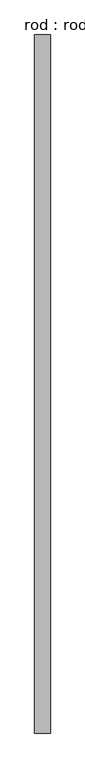
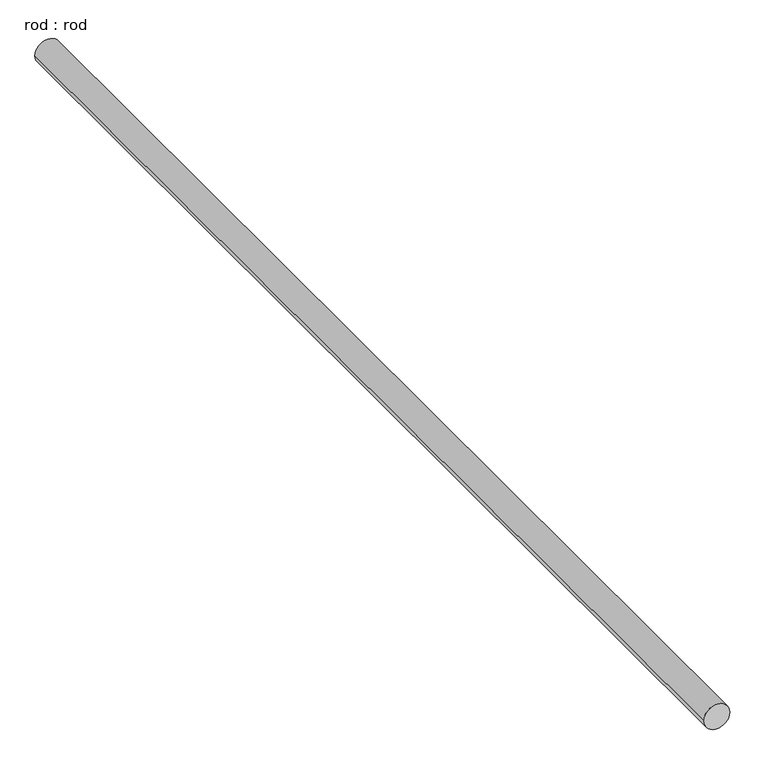
"""IFC4 building model written with IfcOpenShell, lengths in millimetres: proxy geometry, rod : rod."""

import ifcopenshell
import ifcopenshell.guid

model = None  # the IFC model being written
_history = None  # IfcOwnerHistory: only IFC2X3 demands one
_inside = {}  # id of a spatial element -> (the spatial element, [elements in it])
_under = {}  # id of a project, library or spatial element -> (it, [spatial elements below it])
_declared = {}  # id of a project -> (the project, [libraries it declares])
_typed = {}  # id of a type object -> (the type object, [elements of that type])
_made_of = {}  # id of a material, layer set ... -> (it, [elements and type objects made of it])


def new_model(schema):
    """Start an empty IFC model of exactly this schema.

    Asked for "IFC4X3", IfcOpenShell would pick the latest addendum, in which some entities
    have other attributes; the version numbers below select the first issue.
    IFC2X3 requires an IfcOwnerHistory on every rooted entity: one is made here for all.
    """
    global model, _history
    if schema == "IFC4X3":
        model = ifcopenshell.file(schema_version=(4, 3, 0, 0))
    else:
        model = ifcopenshell.file(schema=schema)
    _inside.clear()
    _under.clear()
    _declared.clear()
    _typed.clear()
    _made_of.clear()
    _history = None
    if model.schema == "IFC2X3":
        org = make("IfcOrganization", Name="unknown")
        user = make(
            "IfcPersonAndOrganization",
            ThePerson=make("IfcPerson", FamilyName="unknown"),
            TheOrganization=org,
        )
        app = make(
            "IfcApplication",
            ApplicationDeveloper=org,
            Version="unknown",
            ApplicationFullName="unknown",
            ApplicationIdentifier="unknown",
        )
        _history = make(
            "IfcOwnerHistory",
            OwningUser=user,
            OwningApplication=app,
            ChangeAction="ADDED",
            CreationDate=0,
        )
    return model


def make(cls, **values):
    """One entity of the class cls with the attributes given. An attribute that is None is left unset."""
    return model.create_entity(
        cls, **{name: value for name, value in values.items() if value is not None}
    )


def rooted(cls, **values):
    """An entity with a GlobalId (a new one), such as an element, a storey or a relation."""
    return make(cls, GlobalId=ifcopenshell.guid.new(), OwnerHistory=_history, **values)


def si_unit(unit_type, name, prefix=None):
    """IfcSIUnit, for example si_unit("LENGTHUNIT", "METRE", prefix="MILLI")."""
    return make("IfcSIUnit", UnitType=unit_type, Prefix=prefix, Name=name)


def assignment(units):
    """IfcUnitAssignment: the units of a project."""
    return None if units is None else make("IfcUnitAssignment", Units=units)


def point(xyz):
    """IfcCartesianPoint."""
    return None if xyz is None else make("IfcCartesianPoint", Coordinates=xyz)


def direction(xyz):
    """IfcDirection."""
    return None if xyz is None else make("IfcDirection", DirectionRatios=xyz)


def frame(location, z_axis=None, x_axis=None):
    """IfcAxis2Placement3D, a coordinate frame: its origin and axes. An axis left out is left unset."""
    return make(
        "IfcAxis2Placement3D",
        Location=point(location),
        Axis=direction(z_axis),
        RefDirection=direction(x_axis),
    )


def frame_2d(location, x_axis=None):
    """IfcAxis2Placement2D, a coordinate frame in the plane: its origin and x axis."""
    return make(
        "IfcAxis2Placement2D", Location=point(location), RefDirection=direction(x_axis)
    )


def origin():
    """The frame at (0, 0, 0) with its axes left unset."""
    return frame((0.0, 0.0, 0.0))


def place(relative_to, where):
    """IfcLocalPlacement: puts the frame where relative to a parent placement (None: the world)."""
    return make(
        "IfcLocalPlacement", PlacementRelTo=relative_to, RelativePlacement=where
    )


def context(
    kind, dimensions, precision=None, world=None, true_north=None, identifier=None
):
    """IfcGeometricRepresentationContext, for example the 3D "Model" context."""
    return make(
        "IfcGeometricRepresentationContext",
        ContextIdentifier=identifier,
        ContextType=kind,
        CoordinateSpaceDimension=dimensions,
        Precision=precision,
        WorldCoordinateSystem=world,
        TrueNorth=true_north,
    )


def project(units=None, contexts=None):
    """IfcProject with its units and contexts."""
    return rooted(
        "IfcProject",
        Name="project",
        RepresentationContexts=contexts,
        UnitsInContext=assignment(units),
    )


def spatial(cls, under=None, at=None, **own):
    """A site, building, storey or space (cls), placed at a placement, below another one or the project."""
    s = rooted(cls, ObjectPlacement=at, **own)
    if under is not None:
        _under.setdefault(under.id(), (under, []))[1].append(s)
    return s


def circle_curve(where, radius):
    """IfcCircle in the frame where."""
    return make("IfcCircle", Position=where, Radius=radius)


def trimmed(basis, trim1, trim2, sense, master):
    """IfcTrimmedCurve: the piece of a basis curve between two trims."""
    return make(
        "IfcTrimmedCurve",
        BasisCurve=basis,
        Trim1=trim1,
        Trim2=trim2,
        SenseAgreement=sense,
        MasterRepresentation=master,
    )


def segment(curve, same_sense, transition):
    """IfcCompositeCurveSegment."""
    return make(
        "IfcCompositeCurveSegment",
        Transition=transition,
        SameSense=same_sense,
        ParentCurve=curve,
    )


def composite_curve(segments, self_intersect=None):
    """IfcCompositeCurve: segments joined end to end."""
    return make("IfcCompositeCurve", Segments=segments, SelfIntersect=self_intersect)


def outline(outer, holes=None, kind="AREA"):
    """IfcArbitraryClosedProfileDef: a profile drawn as a closed curve; with holes, ...WithVoids."""
    if holes is None:
        return make("IfcArbitraryClosedProfileDef", ProfileType=kind, OuterCurve=outer)
    return make(
        "IfcArbitraryProfileDefWithVoids",
        ProfileType=kind,
        OuterCurve=outer,
        InnerCurves=holes,
    )


def extrude(swept, where, along, depth):
    """IfcExtrudedAreaSolid: the profile swept, set in the frame where, extruded along a direction by depth."""
    return make(
        "IfcExtrudedAreaSolid",
        SweptArea=swept,
        Position=where,
        ExtrudedDirection=direction(along),
        Depth=depth,
    )


def shape(context_of_items, identifier, shape_type, items):
    """IfcShapeRepresentation: the items that make up one representation, for example the "Body"."""
    return make(
        "IfcShapeRepresentation",
        ContextOfItems=context_of_items,
        RepresentationIdentifier=identifier,
        RepresentationType=shape_type,
        Items=items,
    )


def source(mapping_origin, context_of_items, identifier, shape_type, items):
    """IfcRepresentationMap: a shape defined once, which mapped items show again and again."""
    return make(
        "IfcRepresentationMap",
        MappingOrigin=mapping_origin,
        MappedRepresentation=shape(context_of_items, identifier, shape_type, items),
    )


def transform(
    local_origin,
    x_axis=None,
    y_axis=None,
    z_axis=None,
    scale=None,
    scale2=None,
    scale3=None,
    uniform=True,
):
    """IfcCartesianTransformationOperator3D, or its non-uniform kind. x_axis, y_axis, z_axis: its Axis1, 2, 3."""
    if uniform:
        return make(
            "IfcCartesianTransformationOperator3D",
            Axis1=direction(x_axis),
            Axis2=direction(y_axis),
            LocalOrigin=point(local_origin),
            Scale=scale,
            Axis3=direction(z_axis),
        )
    return make(
        "IfcCartesianTransformationOperator3DnonUniform",
        Axis1=direction(x_axis),
        Axis2=direction(y_axis),
        LocalOrigin=point(local_origin),
        Scale=scale,
        Axis3=direction(z_axis),
        Scale2=scale2,
        Scale3=scale3,
    )


def mapped(mapping_source, mapping_target):
    """IfcMappedItem: shows the shape of a source again, moved by a transform."""
    return make(
        "IfcMappedItem", MappingSource=mapping_source, MappingTarget=mapping_target
    )


def made_of(thing, what):
    """Note that an element or type object is made of a material, layer set ...; save() writes the relation."""
    if what is not None:
        _made_of.setdefault(what.id(), (what, []))[1].append(thing)
    return thing


def element(
    cls,
    number,
    at=None,
    inside=None,
    cuts=None,
    type_object=None,
    material=None,
    context=None,
    identifier="Body",
    shape_type=None,
    held_by="IfcProductDefinitionShape",
    body=None,
    shapes=None,
    **own,
):
    """One element of the class cls, such as IfcWall. Its Tag is "e" and its number.

    at: its placement. inside: the storey or other place that contains it. cuts: it is an
    opening in that element (IfcRelVoidsElement). A single representation is given by context,
    identifier, shape_type and body (its items); several are given by shapes. held_by: the class
    of the entity that holds the representations. save() writes the other relations.
    """
    e = rooted(cls, Tag="e%d" % number, ObjectPlacement=at, **own)
    if body is not None:
        shapes = [shape(context, identifier, shape_type, body)]
    if shapes is not None:
        e.Representation = make(held_by, Representations=shapes)
    if inside is not None:
        _inside.setdefault(inside.id(), (inside, []))[1].append(e)
    if cuts is not None:
        rooted(
            "IfcRelVoidsElement", RelatingBuildingElement=cuts, RelatedOpeningElement=e
        )
    if type_object is not None:
        _typed.setdefault(type_object.id(), (type_object, []))[1].append(e)
    return made_of(e, material)


def aggregate(whole, parts):
    """IfcRelAggregates: a whole, such as a stair, and the parts it consists of."""
    return rooted("IfcRelAggregates", RelatingObject=whole, RelatedObjects=parts)


def save(model, path):
    """Write the relations noted so far, then the file.

    IfcRelAggregates (storeys below a building ...), IfcRelContainedInSpatialStructure (elements
    in a storey), IfcRelDefinesByType, IfcRelAssociatesMaterial and IfcRelDeclares: one each for
    every whole, place, type object, material and project.
    """
    for whole, parts in _under.values():
        aggregate(whole, parts)
    for where, things in _inside.values():
        rooted(
            "IfcRelContainedInSpatialStructure",
            RelatedElements=things,
            RelatingStructure=where,
        )
    for kind, things in _typed.values():
        rooted("IfcRelDefinesByType", RelatedObjects=things, RelatingType=kind)
    for what, things in _made_of.values():
        rooted("IfcRelAssociatesMaterial", RelatedObjects=things, RelatingMaterial=what)
    for by, libraries in _declared.values():
        rooted("IfcRelDeclares", RelatingContext=by, RelatedDefinitions=libraries)
    model.write(path)


def rod_rod_d1b677ea(model_context):
    return source(origin(), model_context, "Body", "SweptSolid", [
        extrude(outline(composite_curve([segment(trimmed(circle_curve(frame_2d((0.0108462, 0.0)), 200.0), [point((0.0108462, 200.0))], [point((0.0108462, -200.0))], False, "CARTESIAN"), True, "CONTINUOUS"), segment(trimmed(circle_curve(frame_2d((0.0108462, 0.0)), 200.0), [point((0.0108462, -200.0))], [point((0.0108462, 200.0))], False, "CARTESIAN"), True, "CONTINUOUS")], self_intersect=False)), frame((0.0, -4812.7069615, 0.0), z_axis=(0.0, 1.0, 0.0), x_axis=(0.0, 0.0, 1.0)), (0.0, 0.0, 1.0), 17810.8711536),
    ])


if __name__ == "__main__":
    model = new_model("IFC4")
    model_context = context("Model", 3, world=origin())
    ifc_project = project(units=[si_unit("LENGTHUNIT", "METRE", prefix="MILLI")], contexts=[model_context])
    site = spatial("IfcSite", under=ifc_project)
    building = spatial("IfcBuilding", under=site)
    placement = place(None, origin())
    rod_rod_shape = rod_rod_d1b677ea(model_context)
    element("IfcBuildingElementProxy", 1, Name="rod : rod", ObjectType="rod : rod", at=placement, inside=building, context=model_context, shape_type="MappedRepresentation", body=[
        mapped(rod_rod_shape, transform((0.0, 0.0, 0.0), x_axis=(1.0, 0.0, 0.0), y_axis=(0.0, 1.0, 0.0), z_axis=(0.0, 0.0, 1.0))),
    ])
    save(model, "model.ifc")

# Revit data of these elements
# Type "rod : rod"
#   Default Elevation = 0
